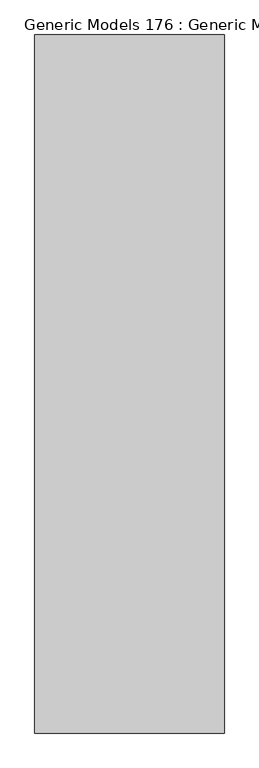
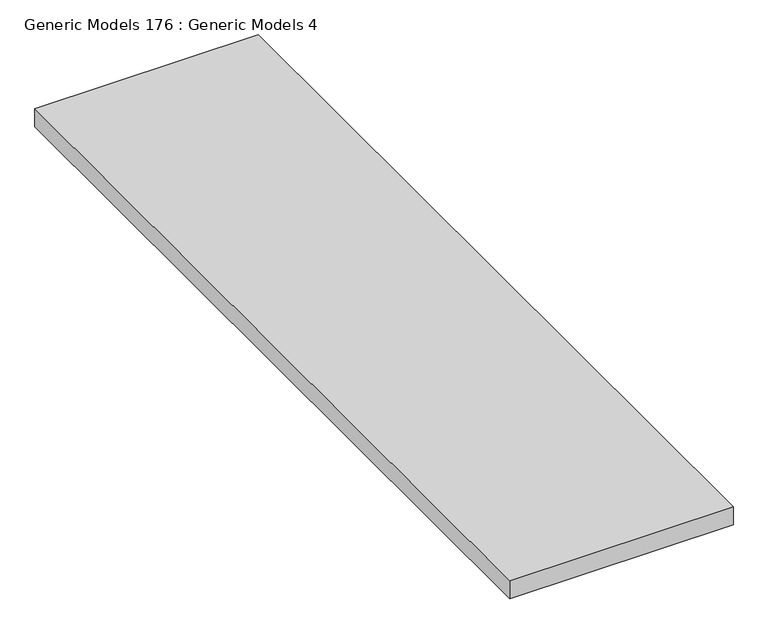
"""IFC4 building model written with IfcOpenShell, lengths in millimetres: proxy geometry, Generic Models 176 : Generic Models 4."""

import ifcopenshell
import ifcopenshell.guid

model = None  # the IFC model being written
_history = None  # IfcOwnerHistory: only IFC2X3 demands one
_inside = {}  # id of a spatial element -> (the spatial element, [elements in it])
_under = {}  # id of a project, library or spatial element -> (it, [spatial elements below it])
_declared = {}  # id of a project -> (the project, [libraries it declares])
_typed = {}  # id of a type object -> (the type object, [elements of that type])
_made_of = {}  # id of a material, layer set ... -> (it, [elements and type objects made of it])


def new_model(schema):
    """Start an empty IFC model of exactly this schema.

    Asked for "IFC4X3", IfcOpenShell would pick the latest addendum, in which some entities
    have other attributes; the version numbers below select the first issue.
    IFC2X3 requires an IfcOwnerHistory on every rooted entity: one is made here for all.
    """
    global model, _history
    if schema == "IFC4X3":
        model = ifcopenshell.file(schema_version=(4, 3, 0, 0))
    else:
        model = ifcopenshell.file(schema=schema)
    _inside.clear()
    _under.clear()
    _declared.clear()
    _typed.clear()
    _made_of.clear()
    _history = None
    if model.schema == "IFC2X3":
        org = make("IfcOrganization", Name="unknown")
        user = make(
            "IfcPersonAndOrganization",
            ThePerson=make("IfcPerson", FamilyName="unknown"),
            TheOrganization=org,
        )
        app = make(
            "IfcApplication",
            ApplicationDeveloper=org,
            Version="unknown",
            ApplicationFullName="unknown",
            ApplicationIdentifier="unknown",
        )
        _history = make(
            "IfcOwnerHistory",
            OwningUser=user,
            OwningApplication=app,
            ChangeAction="ADDED",
            CreationDate=0,
        )
    return model


def make(cls, **values):
    """One entity of the class cls with the attributes given. An attribute that is None is left unset."""
    return model.create_entity(
        cls, **{name: value for name, value in values.items() if value is not None}
    )


def rooted(cls, **values):
    """An entity with a GlobalId (a new one), such as an element, a storey or a relation."""
    return make(cls, GlobalId=ifcopenshell.guid.new(), OwnerHistory=_history, **values)


def si_unit(unit_type, name, prefix=None):
    """IfcSIUnit, for example si_unit("LENGTHUNIT", "METRE", prefix="MILLI")."""
    return make("IfcSIUnit", UnitType=unit_type, Prefix=prefix, Name=name)


def assignment(units):
    """IfcUnitAssignment: the units of a project."""
    return None if units is None else make("IfcUnitAssignment", Units=units)


def point(xyz):
    """IfcCartesianPoint."""
    return None if xyz is None else make("IfcCartesianPoint", Coordinates=xyz)


def direction(xyz):
    """IfcDirection."""
    return None if xyz is None else make("IfcDirection", DirectionRatios=xyz)


def frame(location, z_axis=None, x_axis=None):
    """IfcAxis2Placement3D, a coordinate frame: its origin and axes. An axis left out is left unset."""
    return make(
        "IfcAxis2Placement3D",
        Location=point(location),
        Axis=direction(z_axis),
        RefDirection=direction(x_axis),
    )


def origin():
    """The frame at (0, 0, 0) with its axes left unset."""
    return frame((0.0, 0.0, 0.0))


def place(relative_to, where):
    """IfcLocalPlacement: puts the frame where relative to a parent placement (None: the world)."""
    return make(
        "IfcLocalPlacement", PlacementRelTo=relative_to, RelativePlacement=where
    )


def context(
    kind, dimensions, precision=None, world=None, true_north=None, identifier=None
):
    """IfcGeometricRepresentationContext, for example the 3D "Model" context."""
    return make(
        "IfcGeometricRepresentationContext",
        ContextIdentifier=identifier,
        ContextType=kind,
        CoordinateSpaceDimension=dimensions,
        Precision=precision,
        WorldCoordinateSystem=world,
        TrueNorth=true_north,
    )


def project(units=None, contexts=None):
    """IfcProject with its units and contexts."""
    return rooted(
        "IfcProject",
        Name="project",
        RepresentationContexts=contexts,
        UnitsInContext=assignment(units),
    )


def spatial(cls, under=None, at=None, **own):
    """A site, building, storey or space (cls), placed at a placement, below another one or the project."""
    s = rooted(cls, ObjectPlacement=at, **own)
    if under is not None:
        _under.setdefault(under.id(), (under, []))[1].append(s)
    return s


def polyline(points):
    """IfcPolyline through the points."""
    return make("IfcPolyline", Points=[point(p) for p in points])


def outline(outer, holes=None, kind="AREA"):
    """IfcArbitraryClosedProfileDef: a profile drawn as a closed curve; with holes, ...WithVoids."""
    if holes is None:
        return make("IfcArbitraryClosedProfileDef", ProfileType=kind, OuterCurve=outer)
    return make(
        "IfcArbitraryProfileDefWithVoids",
        ProfileType=kind,
        OuterCurve=outer,
        InnerCurves=holes,
    )


def extrude(swept, where, along, depth):
    """IfcExtrudedAreaSolid: the profile swept, set in the frame where, extruded along a direction by depth."""
    return make(
        "IfcExtrudedAreaSolid",
        SweptArea=swept,
        Position=where,
        ExtrudedDirection=direction(along),
        Depth=depth,
    )


def shape(context_of_items, identifier, shape_type, items):
    """IfcShapeRepresentation: the items that make up one representation, for example the "Body"."""
    return make(
        "IfcShapeRepresentation",
        ContextOfItems=context_of_items,
        RepresentationIdentifier=identifier,
        RepresentationType=shape_type,
        Items=items,
    )


def source(mapping_origin, context_of_items, identifier, shape_type, items):
    """IfcRepresentationMap: a shape defined once, which mapped items show again and again."""
    return make(
        "IfcRepresentationMap",
        MappingOrigin=mapping_origin,
        MappedRepresentation=shape(context_of_items, identifier, shape_type, items),
    )


def transform(
    local_origin,
    x_axis=None,
    y_axis=None,
    z_axis=None,
    scale=None,
    scale2=None,
    scale3=None,
    uniform=True,
):
    """IfcCartesianTransformationOperator3D, or its non-uniform kind. x_axis, y_axis, z_axis: its Axis1, 2, 3."""
    if uniform:
        return make(
            "IfcCartesianTransformationOperator3D",
            Axis1=direction(x_axis),
            Axis2=direction(y_axis),
            LocalOrigin=point(local_origin),
            Scale=scale,
            Axis3=direction(z_axis),
        )
    return make(
        "IfcCartesianTransformationOperator3DnonUniform",
        Axis1=direction(x_axis),
        Axis2=direction(y_axis),
        LocalOrigin=point(local_origin),
        Scale=scale,
        Axis3=direction(z_axis),
        Scale2=scale2,
        Scale3=scale3,
    )


def mapped(mapping_source, mapping_target):
    """IfcMappedItem: shows the shape of a source again, moved by a transform."""
    return make(
        "IfcMappedItem", MappingSource=mapping_source, MappingTarget=mapping_target
    )


def made_of(thing, what):
    """Note that an element or type object is made of a material, layer set ...; save() writes the relation."""
    if what is not None:
        _made_of.setdefault(what.id(), (what, []))[1].append(thing)
    return thing


def element(
    cls,
    number,
    at=None,
    inside=None,
    cuts=None,
    type_object=None,
    material=None,
    context=None,
    identifier="Body",
    shape_type=None,
    held_by="IfcProductDefinitionShape",
    body=None,
    shapes=None,
    **own,
):
    """One element of the class cls, such as IfcWall. Its Tag is "e" and its number.

    at: its placement. inside: the storey or other place that contains it. cuts: it is an
    opening in that element (IfcRelVoidsElement). A single representation is given by context,
    identifier, shape_type and body (its items); several are given by shapes. held_by: the class
    of the entity that holds the representations. save() writes the other relations.
    """
    e = rooted(cls, Tag="e%d" % number, ObjectPlacement=at, **own)
    if body is not None:
        shapes = [shape(context, identifier, shape_type, body)]
    if shapes is not None:
        e.Representation = make(held_by, Representations=shapes)
    if inside is not None:
        _inside.setdefault(inside.id(), (inside, []))[1].append(e)
    if cuts is not None:
        rooted(
            "IfcRelVoidsElement", RelatingBuildingElement=cuts, RelatedOpeningElement=e
        )
    if type_object is not None:
        _typed.setdefault(type_object.id(), (type_object, []))[1].append(e)
    return made_of(e, material)


def aggregate(whole, parts):
    """IfcRelAggregates: a whole, such as a stair, and the parts it consists of."""
    return rooted("IfcRelAggregates", RelatingObject=whole, RelatedObjects=parts)


def save(model, path):
    """Write the relations noted so far, then the file.

    IfcRelAggregates (storeys below a building ...), IfcRelContainedInSpatialStructure (elements
    in a storey), IfcRelDefinesByType, IfcRelAssociatesMaterial and IfcRelDeclares: one each for
    every whole, place, type object, material and project.
    """
    for whole, parts in _under.values():
        aggregate(whole, parts)
    for where, things in _inside.values():
        rooted(
            "IfcRelContainedInSpatialStructure",
            RelatedElements=things,
            RelatingStructure=where,
        )
    for kind, things in _typed.values():
        rooted("IfcRelDefinesByType", RelatedObjects=things, RelatingType=kind)
    for what, things in _made_of.values():
        rooted("IfcRelAssociatesMaterial", RelatedObjects=things, RelatingMaterial=what)
    for by, libraries in _declared.values():
        rooted("IfcRelDeclares", RelatingContext=by, RelatedDefinitions=libraries)
    model.write(path)


def generic_models_176_generic_models_4_0a741b19(model_context):
    return source(origin(), model_context, "Body", "SweptSolid", [
        extrude(outline(polyline([(-6629.5736296, -5493.3230338), (-10037.6722239, -5493.3230338), (-10037.6722239, 7054.2769662), (-6629.5736296, 7054.2769662), (-6629.5736296, -5493.3230338)])), frame((0.0, 0.0, 122511.1484874), z_axis=(0.0, 0.0, 1.0), x_axis=(1.0, 0.0, 0.0)), (0.0, 0.0, 1.0), 292.1),
    ])


if __name__ == "__main__":
    model = new_model("IFC4")
    model_context = context("Model", 3, world=origin())
    ifc_project = project(units=[si_unit("LENGTHUNIT", "METRE", prefix="MILLI")], contexts=[model_context])
    site = spatial("IfcSite", under=ifc_project)
    building = spatial("IfcBuilding", under=site)
    placement = place(None, origin())
    generic_models_176_generic_models_4_shape = generic_models_176_generic_models_4_0a741b19(model_context)
    element("IfcBuildingElementProxy", 1, Name="Generic Models 176 : Generic Models 4", ObjectType="Generic Models 176 : Generic Models 4", at=placement, inside=building, context=model_context, shape_type="MappedRepresentation", body=[
        mapped(generic_models_176_generic_models_4_shape, transform((0.0, 0.0, 0.0), x_axis=(1.0, 0.0, 0.0), y_axis=(0.0, 1.0, 0.0), z_axis=(0.0, 0.0, 1.0))),
    ])
    save(model, "model.ifc")

# Revit data of these elements
# Element 1 (IfcBuildingElementProxy, "Generic Models 176 : Generic Models 4")
#   Materials on its faces: "_COMPACTED GRADE"
# Materials
#   "_COMPACTED GRADE": class "Generic", colour RGB 120 100 58, transparency 0, Cost = 0
